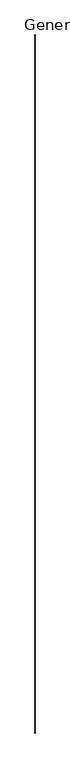
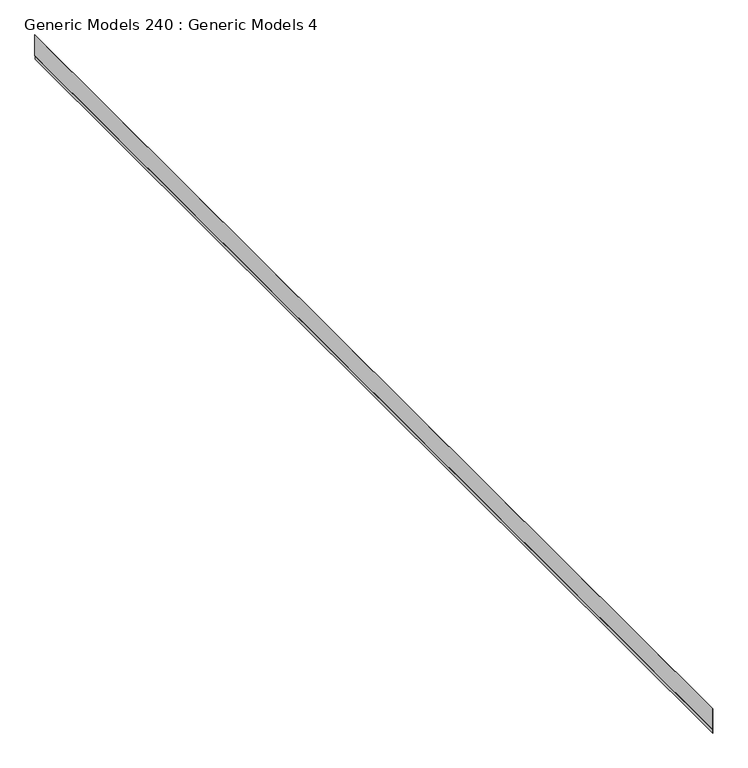
"""IFC4 building model written with IfcOpenShell, lengths in millimetres: proxy geometry, Generic Models 240 : Generic Models 4."""

from ifc_helpers import new_model, si_unit, frame, origin, place, context, project, spatial, polyline, outline, extrude, source, transform, mapped, element, save


def generic_models_240_generic_models_4_168c2a6e(model_context):
    return source(origin(), model_context, "Body", "SweptSolid", [
        extrude(outline(polyline([(126311.4404211, 1638.8605335), (126305.7987003, 1640.9139519), (126258.231851, 1640.9139519), (126258.231851, 1641.7077019), (126305.9386599, 1641.7077019), (126311.5803806, 1639.6542835), (126663.838086, 1639.6542835), (126663.838086, 1638.8605335), (126311.4404211, 1638.8605335)])), frame((0.0, -9028.6126687, 0.0), z_axis=(0.0, 1.0, 0.0), x_axis=(0.0, 0.0, 1.0)), (0.0, 0.0, 1.0), 18643.6),
    ])


if __name__ == "__main__":
    model = new_model("IFC4")
    model_context = context("Model", 3, world=origin())
    ifc_project = project(units=[si_unit("LENGTHUNIT", "METRE", prefix="MILLI")], contexts=[model_context])
    site = spatial("IfcSite", under=ifc_project)
    building = spatial("IfcBuilding", under=site)
    placement = place(None, origin())
    generic_models_240_generic_models_4_shape = generic_models_240_generic_models_4_168c2a6e(model_context)
    element("IfcBuildingElementProxy", 1, Name="Generic Models 240 : Generic Models 4", ObjectType="Generic Models 240 : Generic Models 4", at=placement, inside=building, context=model_context, shape_type="MappedRepresentation", body=[
        mapped(generic_models_240_generic_models_4_shape, transform((0.0, 0.0, 0.0), x_axis=(1.0, 0.0, 0.0), y_axis=(0.0, 1.0, 0.0), z_axis=(0.0, 0.0, 1.0))),
    ])
    save(model, "model.ifc")

# Revit data of these elements
# Element 1 (IfcBuildingElementProxy, "Generic Models 240 : Generic Models 4")
#   Materials on its faces: "_DRAINABLE BUILDING WRAP"
# Materials
#   "_DRAINABLE BUILDING WRAP": class "Generic", colour RGB 67 154 161, transparency 0, Cost = 0
